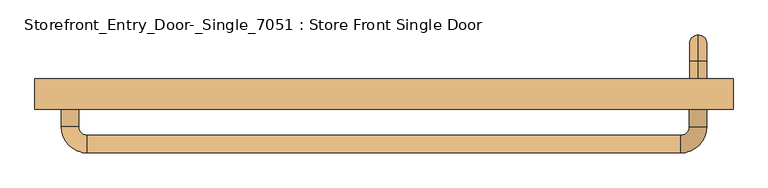
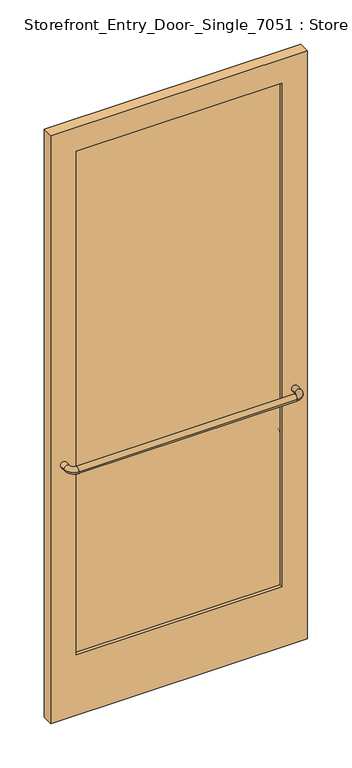
"""IFC4 building model written with IfcOpenShell, lengths in millimetres: door geometry, Storefront_Entry_Door-_Single_7051 : Store Front Single Door."""

import ifcopenshell
import ifcopenshell.guid

model = None  # the IFC model being written
_history = None  # IfcOwnerHistory: only IFC2X3 demands one
_inside = {}  # id of a spatial element -> (the spatial element, [elements in it])
_under = {}  # id of a project, library or spatial element -> (it, [spatial elements below it])
_declared = {}  # id of a project -> (the project, [libraries it declares])
_typed = {}  # id of a type object -> (the type object, [elements of that type])
_made_of = {}  # id of a material, layer set ... -> (it, [elements and type objects made of it])


def new_model(schema):
    """Start an empty IFC model of exactly this schema.

    Asked for "IFC4X3", IfcOpenShell would pick the latest addendum, in which some entities
    have other attributes; the version numbers below select the first issue.
    IFC2X3 requires an IfcOwnerHistory on every rooted entity: one is made here for all.
    """
    global model, _history
    if schema == "IFC4X3":
        model = ifcopenshell.file(schema_version=(4, 3, 0, 0))
    else:
        model = ifcopenshell.file(schema=schema)
    _inside.clear()
    _under.clear()
    _declared.clear()
    _typed.clear()
    _made_of.clear()
    _history = None
    if model.schema == "IFC2X3":
        org = make("IfcOrganization", Name="unknown")
        user = make(
            "IfcPersonAndOrganization",
            ThePerson=make("IfcPerson", FamilyName="unknown"),
            TheOrganization=org,
        )
        app = make(
            "IfcApplication",
            ApplicationDeveloper=org,
            Version="unknown",
            ApplicationFullName="unknown",
            ApplicationIdentifier="unknown",
        )
        _history = make(
            "IfcOwnerHistory",
            OwningUser=user,
            OwningApplication=app,
            ChangeAction="ADDED",
            CreationDate=0,
        )
    return model


def make(cls, **values):
    """One entity of the class cls with the attributes given. An attribute that is None is left unset."""
    return model.create_entity(
        cls, **{name: value for name, value in values.items() if value is not None}
    )


def rooted(cls, **values):
    """An entity with a GlobalId (a new one), such as an element, a storey or a relation."""
    return make(cls, GlobalId=ifcopenshell.guid.new(), OwnerHistory=_history, **values)


def si_unit(unit_type, name, prefix=None):
    """IfcSIUnit, for example si_unit("LENGTHUNIT", "METRE", prefix="MILLI")."""
    return make("IfcSIUnit", UnitType=unit_type, Prefix=prefix, Name=name)


def assignment(units):
    """IfcUnitAssignment: the units of a project."""
    return None if units is None else make("IfcUnitAssignment", Units=units)


def point(xyz):
    """IfcCartesianPoint."""
    return None if xyz is None else make("IfcCartesianPoint", Coordinates=xyz)


def direction(xyz):
    """IfcDirection."""
    return None if xyz is None else make("IfcDirection", DirectionRatios=xyz)


def frame(location, z_axis=None, x_axis=None):
    """IfcAxis2Placement3D, a coordinate frame: its origin and axes. An axis left out is left unset."""
    return make(
        "IfcAxis2Placement3D",
        Location=point(location),
        Axis=direction(z_axis),
        RefDirection=direction(x_axis),
    )


def origin():
    """The frame at (0, 0, 0) with its axes left unset."""
    return frame((0.0, 0.0, 0.0))


def place(relative_to, where):
    """IfcLocalPlacement: puts the frame where relative to a parent placement (None: the world)."""
    return make(
        "IfcLocalPlacement", PlacementRelTo=relative_to, RelativePlacement=where
    )


def context(
    kind, dimensions, precision=None, world=None, true_north=None, identifier=None
):
    """IfcGeometricRepresentationContext, for example the 3D "Model" context."""
    return make(
        "IfcGeometricRepresentationContext",
        ContextIdentifier=identifier,
        ContextType=kind,
        CoordinateSpaceDimension=dimensions,
        Precision=precision,
        WorldCoordinateSystem=world,
        TrueNorth=true_north,
    )


def project(units=None, contexts=None):
    """IfcProject with its units and contexts."""
    return rooted(
        "IfcProject",
        Name="project",
        RepresentationContexts=contexts,
        UnitsInContext=assignment(units),
    )


def spatial(cls, under=None, at=None, **own):
    """A site, building, storey or space (cls), placed at a placement, below another one or the project."""
    s = rooted(cls, ObjectPlacement=at, **own)
    if under is not None:
        _under.setdefault(under.id(), (under, []))[1].append(s)
    return s


def polyline(points):
    """IfcPolyline through the points."""
    return make("IfcPolyline", Points=[point(p) for p in points])


def circle_curve(where, radius):
    """IfcCircle in the frame where."""
    return make("IfcCircle", Position=where, Radius=radius)


def ellipse_curve(where, semi_axis1, semi_axis2):
    """IfcEllipse in the frame where."""
    return make(
        "IfcEllipse", Position=where, SemiAxis1=semi_axis1, SemiAxis2=semi_axis2
    )


def trimmed(basis, trim1, trim2, sense, master):
    """IfcTrimmedCurve: the piece of a basis curve between two trims."""
    return make(
        "IfcTrimmedCurve",
        BasisCurve=basis,
        Trim1=trim1,
        Trim2=trim2,
        SenseAgreement=sense,
        MasterRepresentation=master,
    )


def outline(outer, holes=None, kind="AREA"):
    """IfcArbitraryClosedProfileDef: a profile drawn as a closed curve; with holes, ...WithVoids."""
    if holes is None:
        return make("IfcArbitraryClosedProfileDef", ProfileType=kind, OuterCurve=outer)
    return make(
        "IfcArbitraryProfileDefWithVoids",
        ProfileType=kind,
        OuterCurve=outer,
        InnerCurves=holes,
    )


def extrude(swept, where, along, depth):
    """IfcExtrudedAreaSolid: the profile swept, set in the frame where, extruded along a direction by depth."""
    return make(
        "IfcExtrudedAreaSolid",
        SweptArea=swept,
        Position=where,
        ExtrudedDirection=direction(along),
        Depth=depth,
    )


def shape(context_of_items, identifier, shape_type, items):
    """IfcShapeRepresentation: the items that make up one representation, for example the "Body"."""
    return make(
        "IfcShapeRepresentation",
        ContextOfItems=context_of_items,
        RepresentationIdentifier=identifier,
        RepresentationType=shape_type,
        Items=items,
    )


def source(mapping_origin, context_of_items, identifier, shape_type, items):
    """IfcRepresentationMap: a shape defined once, which mapped items show again and again."""
    return make(
        "IfcRepresentationMap",
        MappingOrigin=mapping_origin,
        MappedRepresentation=shape(context_of_items, identifier, shape_type, items),
    )


def transform(
    local_origin,
    x_axis=None,
    y_axis=None,
    z_axis=None,
    scale=None,
    scale2=None,
    scale3=None,
    uniform=True,
):
    """IfcCartesianTransformationOperator3D, or its non-uniform kind. x_axis, y_axis, z_axis: its Axis1, 2, 3."""
    if uniform:
        return make(
            "IfcCartesianTransformationOperator3D",
            Axis1=direction(x_axis),
            Axis2=direction(y_axis),
            LocalOrigin=point(local_origin),
            Scale=scale,
            Axis3=direction(z_axis),
        )
    return make(
        "IfcCartesianTransformationOperator3DnonUniform",
        Axis1=direction(x_axis),
        Axis2=direction(y_axis),
        LocalOrigin=point(local_origin),
        Scale=scale,
        Axis3=direction(z_axis),
        Scale2=scale2,
        Scale3=scale3,
    )


def mapped(mapping_source, mapping_target):
    """IfcMappedItem: shows the shape of a source again, moved by a transform."""
    return make(
        "IfcMappedItem", MappingSource=mapping_source, MappingTarget=mapping_target
    )


def made_of(thing, what):
    """Note that an element or type object is made of a material, layer set ...; save() writes the relation."""
    if what is not None:
        _made_of.setdefault(what.id(), (what, []))[1].append(thing)
    return thing


def element(
    cls,
    number,
    at=None,
    inside=None,
    cuts=None,
    type_object=None,
    material=None,
    context=None,
    identifier="Body",
    shape_type=None,
    held_by="IfcProductDefinitionShape",
    body=None,
    shapes=None,
    **own,
):
    """One element of the class cls, such as IfcWall. Its Tag is "e" and its number.

    at: its placement. inside: the storey or other place that contains it. cuts: it is an
    opening in that element (IfcRelVoidsElement). A single representation is given by context,
    identifier, shape_type and body (its items); several are given by shapes. held_by: the class
    of the entity that holds the representations. save() writes the other relations.
    """
    e = rooted(cls, Tag="e%d" % number, ObjectPlacement=at, **own)
    if body is not None:
        shapes = [shape(context, identifier, shape_type, body)]
    if shapes is not None:
        e.Representation = make(held_by, Representations=shapes)
    if inside is not None:
        _inside.setdefault(inside.id(), (inside, []))[1].append(e)
    if cuts is not None:
        rooted(
            "IfcRelVoidsElement", RelatingBuildingElement=cuts, RelatedOpeningElement=e
        )
    if type_object is not None:
        _typed.setdefault(type_object.id(), (type_object, []))[1].append(e)
    return made_of(e, material)


def aggregate(whole, parts):
    """IfcRelAggregates: a whole, such as a stair, and the parts it consists of."""
    return rooted("IfcRelAggregates", RelatingObject=whole, RelatedObjects=parts)


def save(model, path):
    """Write the relations noted so far, then the file.

    IfcRelAggregates (storeys below a building ...), IfcRelContainedInSpatialStructure (elements
    in a storey), IfcRelDefinesByType, IfcRelAssociatesMaterial and IfcRelDeclares: one each for
    every whole, place, type object, material and project.
    """
    for whole, parts in _under.values():
        aggregate(whole, parts)
    for where, things in _inside.values():
        rooted(
            "IfcRelContainedInSpatialStructure",
            RelatedElements=things,
            RelatingStructure=where,
        )
    for kind, things in _typed.values():
        rooted("IfcRelDefinesByType", RelatedObjects=things, RelatingType=kind)
    for what, things in _made_of.values():
        rooted("IfcRelAssociatesMaterial", RelatedObjects=things, RelatingMaterial=what)
    for by, libraries in _declared.values():
        rooted("IfcRelDeclares", RelatingContext=by, RelatedDefinitions=libraries)
    model.write(path)


def plane_surface(at):
    """IfcPlane: the flat surface through the origin of the frame at, square to its z axis."""
    return make("IfcPlane", Position=at)


def cylinder_surface(at, radius):
    """IfcCylindricalSurface: all points at the distance radius from the z axis of the frame at."""
    return make("IfcCylindricalSurface", Position=at, Radius=radius)


def revolved_surface(curve, axis_point, axis_direction):
    """IfcSurfaceOfRevolution: the curve turned about the line through axis_point along axis_direction."""
    return make(
        "IfcSurfaceOfRevolution",
        SweptCurve=make("IfcArbitraryOpenProfileDef", ProfileType="CURVE", Curve=curve),
        AxisPosition=make("IfcAxis1Placement", Location=point(axis_point), Axis=direction(axis_direction)),
    )


def advanced_brep(points, edges, surfaces, faces):
    """IfcAdvancedBrep: a solid bounded by faces that lie on surfaces and meet in shared edges.

    An edge is (start, end): straight between two places in points (the first is 0);
    or (start, end, curve); or (start, end, curve, False) where it runs against its curve.
    A face is (place in surfaces, loops), or (place, loops, False) where it looks against
    its surface's normal. A loop lists edges by number (the first is 1), with a minus sign
    where the edge is run from its end to its start. The first loop is the outer one.
    """
    corners = [point(p) for p in points]
    vertices = [make("IfcVertexPoint", VertexGeometry=c) for c in corners]
    made = []
    for start, end, *more in edges:
        made.append(
            make(
                "IfcEdgeCurve",
                EdgeStart=vertices[start],
                EdgeEnd=vertices[end],
                EdgeGeometry=more[0] if more else make("IfcPolyline", Points=[corners[start], corners[end]]),
                SameSense=more[1] if len(more) > 1 else True,
            )
        )
    hull = []
    for where, loops, *sense in faces:
        bounds = []
        for j, loop in enumerate(loops):
            ring = [make("IfcOrientedEdge", EdgeElement=made[abs(k) - 1], Orientation=k > 0) for k in loop]
            bounds.append(
                make(
                    "IfcFaceOuterBound" if j == 0 else "IfcFaceBound",
                    Bound=make("IfcEdgeLoop", EdgeList=ring),
                    Orientation=True,
                )
            )
        hull.append(make("IfcAdvancedFace", Bounds=bounds, FaceSurface=surfaces[where], SameSense=sense[0] if sense else True))
    return make("IfcAdvancedBrep", Outer=make("IfcClosedShell", CfsFaces=hull))


def storefront_entry_door_single_7051_store_front_single_door_83381969(model_context):
    return source(origin(), model_context, "Body", "SolidModel", [
        advanced_brep(
        [(457.2, 50.8, 1054.1), (457.2, 50.8, 1079.5), (457.2, 76.2, 1054.1), (457.2, 76.2, 1079.5), (457.2, 114.3, 1041.4), (457.2, 88.9, 1041.4), (457.2, 88.9, 863.6), (457.2, 114.3, 863.6), (457.2, 76.2, 825.5), (457.2, 76.2, 850.9), (457.2, 50.8, 850.9), (457.2, 50.8, 825.5)],
        [
            (0, 1, circle_curve(frame((457.2, 50.8, 1066.8), z_axis=(0.0, -1.0, 0.0), x_axis=(0.0, 0.0, 1.0)), 12.7)),
            (1, 0, circle_curve(frame((457.2, 50.8, 1066.8), z_axis=(0.0, -1.0, 0.0), x_axis=(0.0, 0.0, 1.0)), 12.7)),
            (0, 2),
            (2, 3, circle_curve(frame((457.2, 76.2, 1066.8), z_axis=(0.0, -1.0, 0.0), x_axis=(0.0, 0.0, 1.0)), 12.7)),
            (3, 1),
            (3, 2, circle_curve(frame((457.2, 76.2, 1066.8), z_axis=(0.0, -1.0, 0.0), x_axis=(0.0, 0.0, 1.0)), 12.7)),
            (4, 3, circle_curve(frame((457.2, 76.2, 1041.4), z_axis=(1.0, 0.0, 0.0), x_axis=(0.0, 0.0, 1.0)), 38.1)),
            (2, 5, circle_curve(frame((457.2, 76.2, 1041.4), z_axis=(-1.0, 0.0, 0.0), x_axis=(0.0, 0.0, 1.0)), 12.7)),
            (5, 4, circle_curve(frame((457.2, 101.6, 1041.4), z_axis=(0.0, 0.0, 1.0), x_axis=(0.0, 1.0, 0.0)), 12.7)),
            (4, 5, circle_curve(frame((457.2, 101.6, 1041.4), z_axis=(0.0, 0.0, 1.0), x_axis=(0.0, 1.0, 0.0)), 12.7)),
            (5, 6),
            (6, 7, circle_curve(frame((457.2, 101.6, 863.6), z_axis=(0.0, 0.0, 1.0), x_axis=(0.0, 1.0, 0.0)), 12.7)),
            (7, 4),
            (7, 6, circle_curve(frame((457.2, 101.6, 863.6), z_axis=(0.0, 0.0, 1.0), x_axis=(0.0, 1.0, 0.0)), 12.7)),
            (8, 7, circle_curve(frame((457.2, 76.2, 863.6), z_axis=(1.0, 0.0, 0.0), x_axis=(0.0, 1.0, 0.0)), 38.1)),
            (6, 9, circle_curve(frame((457.2, 76.2, 863.6), z_axis=(-1.0, 0.0, 0.0), x_axis=(0.0, 1.0, 0.0)), 12.7)),
            (9, 8, circle_curve(frame((457.2, 76.2, 838.2), z_axis=(0.0, 1.0, 0.0), x_axis=(0.0, 0.0, -1.0)), 12.7)),
            (8, 9, circle_curve(frame((457.2, 76.2, 838.2), z_axis=(0.0, 1.0, 0.0), x_axis=(0.0, 0.0, -1.0)), 12.7)),
            (10, 11, circle_curve(frame((457.2, 50.8, 838.2), z_axis=(0.0, -1.0, 0.0), x_axis=(0.0, 0.0, -1.0)), 12.7)),
            (11, 10, circle_curve(frame((457.2, 50.8, 838.2), z_axis=(0.0, -1.0, 0.0), x_axis=(0.0, 0.0, -1.0)), 12.7)),
            (9, 10),
            (11, 8),
        ],
        [
            plane_surface(frame((457.2, 50.8, 1066.8), z_axis=(0.0, -1.0, 0.0), x_axis=(1.0, 0.0, 0.0))),
            cylinder_surface(frame((457.2, 50.8, 1066.8), z_axis=(0.0, -1.0, 0.0), x_axis=(0.0, 0.0, 1.0)), 12.7),
            revolved_surface(trimmed(ellipse_curve(frame((457.2, 76.2, 1066.8), z_axis=(0.0, -1.0, 0.0), x_axis=(0.0, 0.0, 1.0)), 12.7, 12.7), [point((457.2, 76.2, 1054.1))], [point((457.2, 76.2, 1079.5))], True, "CARTESIAN"), (457.2, 76.2, 1041.4), (-1.0, 0.0, 0.0)),
            revolved_surface(trimmed(ellipse_curve(frame((457.2, 76.2, 1066.8), z_axis=(0.0, -1.0, 0.0), x_axis=(0.0, 0.0, 1.0)), 12.7, 12.7), [point((457.2, 76.2, 1079.5))], [point((457.2, 76.2, 1054.1))], True, "CARTESIAN"), (457.2, 76.2, 1041.4), (-1.0, 0.0, 0.0)),
            cylinder_surface(frame((457.2, 101.6, 1041.4), z_axis=(0.0, 0.0, 1.0), x_axis=(0.0, 1.0, 0.0)), 12.7),
            revolved_surface(trimmed(ellipse_curve(frame((457.2, 101.6, 863.6), z_axis=(0.0, 0.0, 1.0), x_axis=(0.0, 1.0, 0.0)), 12.7, 12.7), [point((457.2, 88.9, 863.6))], [point((457.2, 114.3, 863.6))], True, "CARTESIAN"), (457.2, 76.2, 863.6), (-1.0, 0.0, 0.0)),
            revolved_surface(trimmed(ellipse_curve(frame((457.2, 101.6, 863.6), z_axis=(0.0, 0.0, 1.0), x_axis=(0.0, 1.0, 0.0)), 12.7, 12.7), [point((457.2, 114.3, 863.6))], [point((457.2, 88.9, 863.6))], True, "CARTESIAN"), (457.2, 76.2, 863.6), (-1.0, 0.0, 0.0)),
            plane_surface(frame((457.2, 50.8, 838.2), z_axis=(0.0, -1.0, 0.0), x_axis=(1.0, 0.0, 0.0))),
            cylinder_surface(frame((457.2, 76.2, 838.2), z_axis=(0.0, 1.0, 0.0), x_axis=(0.0, 0.0, -1.0)), 12.7),
        ],
        [
            (0, [[1, 2]]),
            (1, [[-1, 3, 4, 5]]),
            (1, [[-2, -5, 6, -3]]),
            (2, [[7, -4, 8, 9]]),
            (3, [[-8, -6, -7, 10]]),
            (4, [[-9, 11, 12, 13]]),
            (4, [[-10, -13, 14, -11]]),
            (5, [[15, -12, 16, 17]]),
            (6, [[-16, -14, -15, 18]]),
            (7, [[19, 20]]),
            (8, [[-17, 21, -20, 22]]),
            (8, [[-18, -22, -19, -21]]),
        ],
    ),
        advanced_brep(
        [(444.5, 6.35, 1066.8), (469.9, 6.35, 1066.8), (444.5, -19.05, 1066.8), (469.9, -19.05, 1066.8), (431.8, -57.15, 1066.8), (431.8, -31.75, 1066.8), (-431.8, -31.75, 1066.8), (-431.8, -57.15, 1066.8), (-469.9, -19.05, 1066.8), (-444.5, -19.05, 1066.8), (-444.5, 6.35, 1066.8), (-469.9, 6.35, 1066.8)],
        [
            (0, 1, circle_curve(frame((457.2, 6.35, 1066.8), z_axis=(0.0, 1.0, 0.0), x_axis=(1.0, 0.0, 0.0)), 12.7)),
            (1, 0, circle_curve(frame((457.2, 6.35, 1066.8), z_axis=(0.0, 1.0, 0.0), x_axis=(1.0, 0.0, 0.0)), 12.7)),
            (0, 2),
            (2, 3, circle_curve(frame((457.2, -19.05, 1066.8), z_axis=(0.0, 1.0, 0.0), x_axis=(1.0, 0.0, 0.0)), 12.7)),
            (3, 1),
            (3, 2, circle_curve(frame((457.2, -19.05, 1066.8), z_axis=(0.0, 1.0, 0.0), x_axis=(1.0, 0.0, 0.0)), 12.7)),
            (4, 3, circle_curve(frame((431.8, -19.05, 1066.8), z_axis=(0.0, 0.0, 1.0), x_axis=(1.0, 0.0, 0.0)), 38.1)),
            (2, 5, circle_curve(frame((431.8, -19.05, 1066.8), z_axis=(0.0, 0.0, -1.0), x_axis=(1.0, 0.0, 0.0)), 12.7)),
            (5, 4, circle_curve(frame((431.8, -44.45, 1066.8), z_axis=(1.0, 0.0, 0.0), x_axis=(0.0, -1.0, 0.0)), 12.7)),
            (4, 5, circle_curve(frame((431.8, -44.45, 1066.8), z_axis=(1.0, 0.0, 0.0), x_axis=(0.0, -1.0, 0.0)), 12.7)),
            (5, 6),
            (6, 7, circle_curve(frame((-431.8, -44.45, 1066.8), z_axis=(1.0, 0.0, 0.0), x_axis=(0.0, -1.0, 0.0)), 12.7)),
            (7, 4),
            (7, 6, circle_curve(frame((-431.8, -44.45, 1066.8), z_axis=(1.0, 0.0, 0.0), x_axis=(0.0, -1.0, 0.0)), 12.7)),
            (8, 7, circle_curve(frame((-431.8, -19.05, 1066.8), z_axis=(0.0, 0.0, 1.0), x_axis=(0.0, -1.0, 0.0)), 38.1)),
            (6, 9, circle_curve(frame((-431.8, -19.05, 1066.8), z_axis=(0.0, 0.0, -1.0), x_axis=(0.0, -1.0, 0.0)), 12.7)),
            (9, 8, circle_curve(frame((-457.2, -19.05, 1066.8), z_axis=(0.0, -1.0, 0.0), x_axis=(-1.0, 0.0, 0.0)), 12.7)),
            (8, 9, circle_curve(frame((-457.2, -19.05, 1066.8), z_axis=(0.0, -1.0, 0.0), x_axis=(-1.0, 0.0, 0.0)), 12.7)),
            (10, 11, circle_curve(frame((-457.2, 6.35, 1066.8), z_axis=(0.0, 1.0, 0.0), x_axis=(-1.0, 0.0, 0.0)), 12.7)),
            (11, 10, circle_curve(frame((-457.2, 6.35, 1066.8), z_axis=(0.0, 1.0, 0.0), x_axis=(-1.0, 0.0, 0.0)), 12.7)),
            (9, 10),
            (11, 8),
        ],
        [
            plane_surface(frame((457.2, 6.35, 1066.8), z_axis=(0.0, 1.0, 0.0), x_axis=(0.0, 0.0, 1.0))),
            cylinder_surface(frame((457.2, 6.35, 1066.8), z_axis=(0.0, 1.0, 0.0), x_axis=(1.0, 0.0, 0.0)), 12.7),
            revolved_surface(trimmed(ellipse_curve(frame((457.2, -19.05, 1066.8), z_axis=(0.0, 1.0, 0.0), x_axis=(1.0, 0.0, 0.0)), 12.7, 12.7), [point((444.5, -19.05, 1066.8))], [point((469.9, -19.05, 1066.8))], True, "CARTESIAN"), (431.8, -19.05, 1066.8), (0.0, 0.0, -1.0)),
            revolved_surface(trimmed(ellipse_curve(frame((457.2, -19.05, 1066.8), z_axis=(0.0, 1.0, 0.0), x_axis=(1.0, 0.0, 0.0)), 12.7, 12.7), [point((469.9, -19.05, 1066.8))], [point((444.5, -19.05, 1066.8))], True, "CARTESIAN"), (431.8, -19.05, 1066.8), (0.0, 0.0, -1.0)),
            cylinder_surface(frame((431.8, -44.45, 1066.8), z_axis=(1.0, 0.0, 0.0), x_axis=(0.0, -1.0, 0.0)), 12.7),
            revolved_surface(trimmed(ellipse_curve(frame((-431.8, -44.45, 1066.8), z_axis=(1.0, 0.0, 0.0), x_axis=(0.0, -1.0, 0.0)), 12.7, 12.7), [point((-431.8, -31.75, 1066.8))], [point((-431.8, -57.15, 1066.8))], True, "CARTESIAN"), (-431.8, -19.05, 1066.8), (0.0, 0.0, -1.0)),
            revolved_surface(trimmed(ellipse_curve(frame((-431.8, -44.45, 1066.8), z_axis=(1.0, 0.0, 0.0), x_axis=(0.0, -1.0, 0.0)), 12.7, 12.7), [point((-431.8, -57.15, 1066.8))], [point((-431.8, -31.75, 1066.8))], True, "CARTESIAN"), (-431.8, -19.05, 1066.8), (0.0, 0.0, -1.0)),
            plane_surface(frame((-457.2, 6.35, 1066.8), z_axis=(0.0, 1.0, 0.0), x_axis=(0.0, 0.0, 1.0))),
            cylinder_surface(frame((-457.2, -19.05, 1066.8), z_axis=(0.0, -1.0, 0.0), x_axis=(-1.0, 0.0, 0.0)), 12.7),
        ],
        [
            (0, [[1, 2]]),
            (1, [[-1, 3, 4, 5]]),
            (1, [[-2, -5, 6, -3]]),
            (2, [[7, -4, 8, 9]]),
            (3, [[-8, -6, -7, 10]]),
            (4, [[-9, 11, 12, 13]]),
            (4, [[-10, -13, 14, -11]]),
            (5, [[15, -12, 16, 17]]),
            (6, [[-16, -14, -15, 18]]),
            (7, [[19, 20]]),
            (8, [[-17, 21, -20, 22]]),
            (8, [[-18, -22, -19, -21]]),
        ],
    ),
        extrude(outline(polyline([(406.4, 19.05), (-406.4, 19.05), (-406.4, 38.1), (406.4, 38.1), (406.4, 19.05)])), frame((0.0, 0.0, 254.0), z_axis=(0.0, 0.0, 1.0), x_axis=(1.0, 0.0, 0.0)), (0.0, 0.0, 1.0), 2105.025),
        extrude(outline(polyline([(2460.625, 508.0), (2460.625, -508.0), (0.0, -508.0), (0.0, 508.0), (2460.625, 508.0)]), holes=[polyline([(2359.025, -406.4), (2359.025, 406.4), (254.0, 406.4), (254.0, -406.4), (2359.025, -406.4)])]), frame((0.0, 6.35, 0.0), z_axis=(0.0, 1.0, 0.0), x_axis=(0.0, 0.0, 1.0)), (0.0, 0.0, 1.0), 44.45),
    ])


if __name__ == "__main__":
    model = new_model("IFC4")
    model_context = context("Model", 3, world=origin())
    ifc_project = project(units=[si_unit("LENGTHUNIT", "METRE", prefix="MILLI")], contexts=[model_context])
    site = spatial("IfcSite", under=ifc_project)
    building = spatial("IfcBuilding", under=site)
    placement = place(None, origin())
    storefront_entry_door_single_7051_store_front_single_door_shape = storefront_entry_door_single_7051_store_front_single_door_83381969(model_context)
    element("IfcDoor", 1, ObjectType="Storefront_Entry_Door-_Single_7051 : Store Front Single Door", at=placement, inside=building, context=model_context, shape_type="MappedRepresentation", body=[
        mapped(storefront_entry_door_single_7051_store_front_single_door_shape, transform((0.0, 0.0, 0.0), x_axis=(1.0, 0.0, 0.0), y_axis=(0.0, 1.0, 0.0), z_axis=(0.0, 0.0, 1.0))),
    ])
    save(model, "model.ifc")

# Revit data of these elements
# Type "Storefront_Entry_Door-_Single_7051 : Store Front Single Door"
#   Type Comments = "TEMPERED GLAZING"
#   Type Mark = "19"
#   Assembly Code = "B2030110"
#   Analytic Construction = "<None>"
#   Top Rail = 0' - 4"
#   Side Rail = 0' - 4"
#   Reporting Width [instance default] = 4' - 2"
#   Rail Height AFF = 3' - 6"
#   Offset = 0' - 2"
#   Door Width [instance default] = 4' - 2"
#   Bottom Rail Width = 0' - 10"
#   Material = Metal - Aluminum
#   Glazing Material = Glass
#   Function = (empty or 0)
# Element 1 (IfcDoor, "Storefront_Entry_Door-_Single_7051 : Store Front Single Door")
#   Reporting Width = 3' - 4"
#   Door Width = 3' - 4"
#   Materials on its faces: "Metal - Aluminum", "Glass"
# Materials
#   "Metal - Aluminum": class "Metal", colour RGB 247 247 247, transparency 0
#   "Glass": class "Glass", colour RGB 218 227 224, transparency 0.85, Description = "Soda Lime Glass", Cost = 0
